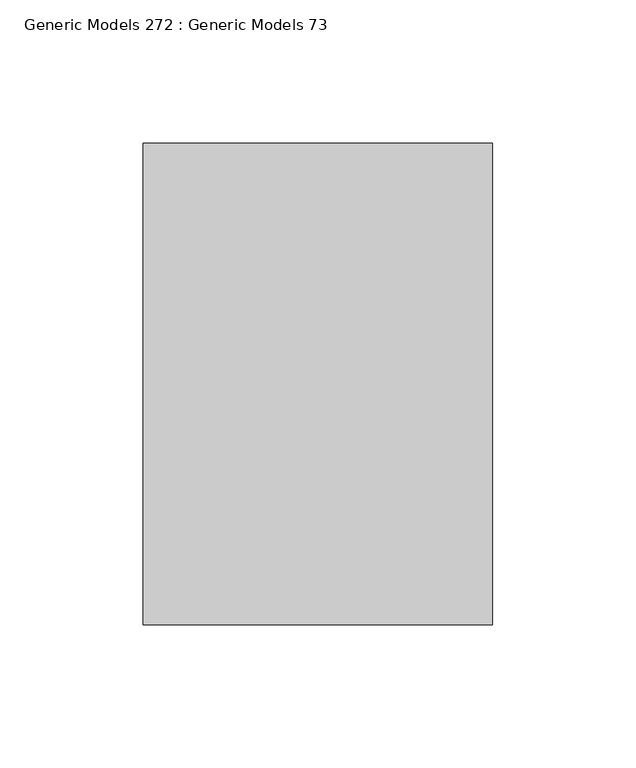
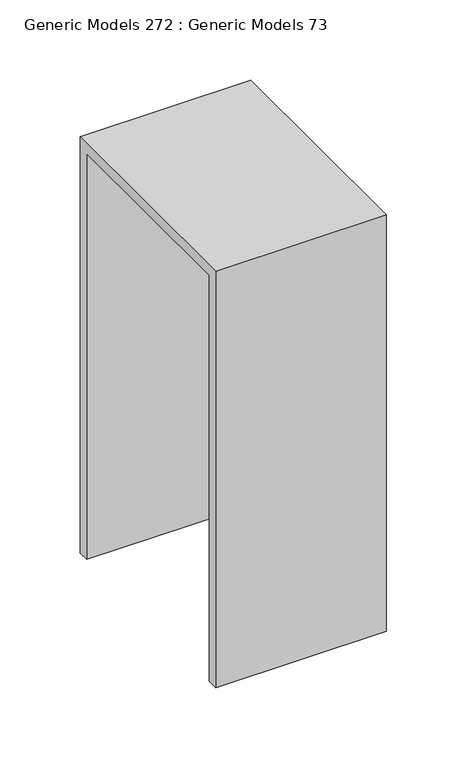
"""IFC4 building model written with IfcOpenShell, lengths in millimetres: proxy geometry, Generic Models 272 : Generic Models 73."""

from ifc_helpers import new_model, si_unit, frame, origin, place, context, project, spatial, polyline, outline, extrude, source, transform, mapped, element, save


def generic_models_272_generic_models_73_2b91d6a2(model_context):
    return source(origin(), model_context, "Body", "SweptSolid", [
        extrude(outline(polyline([(36483.6207942, 271789.525), (36331.2207942, 271789.525), (36331.2207942, 271481.55), (36323.2832942, 271481.55), (36323.2832942, 271797.4625), (36491.5582942, 271797.4625), (36491.5582942, 271481.55), (36483.6207942, 271481.55), (36483.6207942, 271789.525)])), frame((31930.9715778, 0.0, 0.0), z_axis=(1.0, 0.0, 0.0), x_axis=(0.0, 1.0, 0.0)), (0.0, 0.0, 1.0), 122.2375),
    ])


if __name__ == "__main__":
    model = new_model("IFC4")
    model_context = context("Model", 3, world=origin())
    ifc_project = project(units=[si_unit("LENGTHUNIT", "METRE", prefix="MILLI")], contexts=[model_context])
    site = spatial("IfcSite", under=ifc_project)
    building = spatial("IfcBuilding", under=site)
    placement = place(None, origin())
    generic_models_272_generic_models_73_shape = generic_models_272_generic_models_73_2b91d6a2(model_context)
    element("IfcBuildingElementProxy", 1, Name="Generic Models 272 : Generic Models 73", ObjectType="Generic Models 272 : Generic Models 73", at=placement, inside=building, context=model_context, shape_type="MappedRepresentation", body=[
        mapped(generic_models_272_generic_models_73_shape, transform((0.0, 0.0, 0.0), x_axis=(1.0, 0.0, 0.0), y_axis=(0.0, 1.0, 0.0), z_axis=(0.0, 0.0, 1.0))),
    ])
    save(model, "model.ifc")

# Revit data of these elements
# Element 1 (IfcBuildingElementProxy, "Generic Models 272 : Generic Models 73")
#   Materials on its faces: "5/16 GALV. PLATE"
# Materials
#   "5/16 GALV. PLATE": class "Metal", colour RGB 199 199 199, transparency 0, Description = "Carbon steel", Cost = 0
